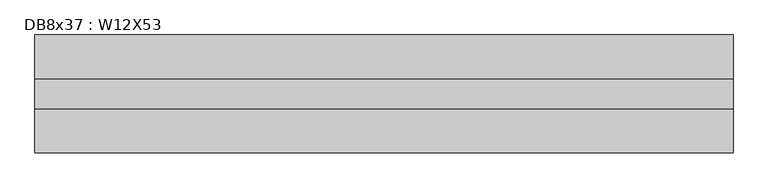
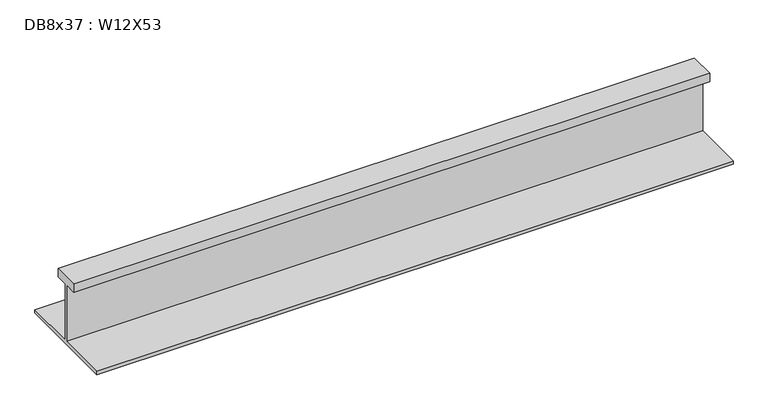
"""IFC4 building model written with IfcOpenShell, lengths in millimetres: beam geometry, DB8x37 : W12X53."""

import ifcopenshell
import ifcopenshell.guid

model = None  # the IFC model being written
_history = None  # IfcOwnerHistory: only IFC2X3 demands one
_inside = {}  # id of a spatial element -> (the spatial element, [elements in it])
_under = {}  # id of a project, library or spatial element -> (it, [spatial elements below it])
_declared = {}  # id of a project -> (the project, [libraries it declares])
_typed = {}  # id of a type object -> (the type object, [elements of that type])
_made_of = {}  # id of a material, layer set ... -> (it, [elements and type objects made of it])


def new_model(schema):
    """Start an empty IFC model of exactly this schema.

    Asked for "IFC4X3", IfcOpenShell would pick the latest addendum, in which some entities
    have other attributes; the version numbers below select the first issue.
    IFC2X3 requires an IfcOwnerHistory on every rooted entity: one is made here for all.
    """
    global model, _history
    if schema == "IFC4X3":
        model = ifcopenshell.file(schema_version=(4, 3, 0, 0))
    else:
        model = ifcopenshell.file(schema=schema)
    _inside.clear()
    _under.clear()
    _declared.clear()
    _typed.clear()
    _made_of.clear()
    _history = None
    if model.schema == "IFC2X3":
        org = make("IfcOrganization", Name="unknown")
        user = make(
            "IfcPersonAndOrganization",
            ThePerson=make("IfcPerson", FamilyName="unknown"),
            TheOrganization=org,
        )
        app = make(
            "IfcApplication",
            ApplicationDeveloper=org,
            Version="unknown",
            ApplicationFullName="unknown",
            ApplicationIdentifier="unknown",
        )
        _history = make(
            "IfcOwnerHistory",
            OwningUser=user,
            OwningApplication=app,
            ChangeAction="ADDED",
            CreationDate=0,
        )
    return model


def make(cls, **values):
    """One entity of the class cls with the attributes given. An attribute that is None is left unset."""
    return model.create_entity(
        cls, **{name: value for name, value in values.items() if value is not None}
    )


def rooted(cls, **values):
    """An entity with a GlobalId (a new one), such as an element, a storey or a relation."""
    return make(cls, GlobalId=ifcopenshell.guid.new(), OwnerHistory=_history, **values)


def si_unit(unit_type, name, prefix=None):
    """IfcSIUnit, for example si_unit("LENGTHUNIT", "METRE", prefix="MILLI")."""
    return make("IfcSIUnit", UnitType=unit_type, Prefix=prefix, Name=name)


def assignment(units):
    """IfcUnitAssignment: the units of a project."""
    return None if units is None else make("IfcUnitAssignment", Units=units)


def point(xyz):
    """IfcCartesianPoint."""
    return None if xyz is None else make("IfcCartesianPoint", Coordinates=xyz)


def direction(xyz):
    """IfcDirection."""
    return None if xyz is None else make("IfcDirection", DirectionRatios=xyz)


def frame(location, z_axis=None, x_axis=None):
    """IfcAxis2Placement3D, a coordinate frame: its origin and axes. An axis left out is left unset."""
    return make(
        "IfcAxis2Placement3D",
        Location=point(location),
        Axis=direction(z_axis),
        RefDirection=direction(x_axis),
    )


def origin():
    """The frame at (0, 0, 0) with its axes left unset."""
    return frame((0.0, 0.0, 0.0))


def place(relative_to, where):
    """IfcLocalPlacement: puts the frame where relative to a parent placement (None: the world)."""
    return make(
        "IfcLocalPlacement", PlacementRelTo=relative_to, RelativePlacement=where
    )


def context(
    kind, dimensions, precision=None, world=None, true_north=None, identifier=None
):
    """IfcGeometricRepresentationContext, for example the 3D "Model" context."""
    return make(
        "IfcGeometricRepresentationContext",
        ContextIdentifier=identifier,
        ContextType=kind,
        CoordinateSpaceDimension=dimensions,
        Precision=precision,
        WorldCoordinateSystem=world,
        TrueNorth=true_north,
    )


def project(units=None, contexts=None):
    """IfcProject with its units and contexts."""
    return rooted(
        "IfcProject",
        Name="project",
        RepresentationContexts=contexts,
        UnitsInContext=assignment(units),
    )


def spatial(cls, under=None, at=None, **own):
    """A site, building, storey or space (cls), placed at a placement, below another one or the project."""
    s = rooted(cls, ObjectPlacement=at, **own)
    if under is not None:
        _under.setdefault(under.id(), (under, []))[1].append(s)
    return s


def polyline(points):
    """IfcPolyline through the points."""
    return make("IfcPolyline", Points=[point(p) for p in points])


def outline(outer, holes=None, kind="AREA"):
    """IfcArbitraryClosedProfileDef: a profile drawn as a closed curve; with holes, ...WithVoids."""
    if holes is None:
        return make("IfcArbitraryClosedProfileDef", ProfileType=kind, OuterCurve=outer)
    return make(
        "IfcArbitraryProfileDefWithVoids",
        ProfileType=kind,
        OuterCurve=outer,
        InnerCurves=holes,
    )


def extrude(swept, where, along, depth):
    """IfcExtrudedAreaSolid: the profile swept, set in the frame where, extruded along a direction by depth."""
    return make(
        "IfcExtrudedAreaSolid",
        SweptArea=swept,
        Position=where,
        ExtrudedDirection=direction(along),
        Depth=depth,
    )


def shape(context_of_items, identifier, shape_type, items):
    """IfcShapeRepresentation: the items that make up one representation, for example the "Body"."""
    return make(
        "IfcShapeRepresentation",
        ContextOfItems=context_of_items,
        RepresentationIdentifier=identifier,
        RepresentationType=shape_type,
        Items=items,
    )


def source(mapping_origin, context_of_items, identifier, shape_type, items):
    """IfcRepresentationMap: a shape defined once, which mapped items show again and again."""
    return make(
        "IfcRepresentationMap",
        MappingOrigin=mapping_origin,
        MappedRepresentation=shape(context_of_items, identifier, shape_type, items),
    )


def transform(
    local_origin,
    x_axis=None,
    y_axis=None,
    z_axis=None,
    scale=None,
    scale2=None,
    scale3=None,
    uniform=True,
):
    """IfcCartesianTransformationOperator3D, or its non-uniform kind. x_axis, y_axis, z_axis: its Axis1, 2, 3."""
    if uniform:
        return make(
            "IfcCartesianTransformationOperator3D",
            Axis1=direction(x_axis),
            Axis2=direction(y_axis),
            LocalOrigin=point(local_origin),
            Scale=scale,
            Axis3=direction(z_axis),
        )
    return make(
        "IfcCartesianTransformationOperator3DnonUniform",
        Axis1=direction(x_axis),
        Axis2=direction(y_axis),
        LocalOrigin=point(local_origin),
        Scale=scale,
        Axis3=direction(z_axis),
        Scale2=scale2,
        Scale3=scale3,
    )


def mapped(mapping_source, mapping_target):
    """IfcMappedItem: shows the shape of a source again, moved by a transform."""
    return make(
        "IfcMappedItem", MappingSource=mapping_source, MappingTarget=mapping_target
    )


def made_of(thing, what):
    """Note that an element or type object is made of a material, layer set ...; save() writes the relation."""
    if what is not None:
        _made_of.setdefault(what.id(), (what, []))[1].append(thing)
    return thing


def element(
    cls,
    number,
    at=None,
    inside=None,
    cuts=None,
    type_object=None,
    material=None,
    context=None,
    identifier="Body",
    shape_type=None,
    held_by="IfcProductDefinitionShape",
    body=None,
    shapes=None,
    **own,
):
    """One element of the class cls, such as IfcWall. Its Tag is "e" and its number.

    at: its placement. inside: the storey or other place that contains it. cuts: it is an
    opening in that element (IfcRelVoidsElement). A single representation is given by context,
    identifier, shape_type and body (its items); several are given by shapes. held_by: the class
    of the entity that holds the representations. save() writes the other relations.
    """
    e = rooted(cls, Tag="e%d" % number, ObjectPlacement=at, **own)
    if body is not None:
        shapes = [shape(context, identifier, shape_type, body)]
    if shapes is not None:
        e.Representation = make(held_by, Representations=shapes)
    if inside is not None:
        _inside.setdefault(inside.id(), (inside, []))[1].append(e)
    if cuts is not None:
        rooted(
            "IfcRelVoidsElement", RelatingBuildingElement=cuts, RelatedOpeningElement=e
        )
    if type_object is not None:
        _typed.setdefault(type_object.id(), (type_object, []))[1].append(e)
    return made_of(e, material)


def aggregate(whole, parts):
    """IfcRelAggregates: a whole, such as a stair, and the parts it consists of."""
    return rooted("IfcRelAggregates", RelatingObject=whole, RelatedObjects=parts)


def save(model, path):
    """Write the relations noted so far, then the file.

    IfcRelAggregates (storeys below a building ...), IfcRelContainedInSpatialStructure (elements
    in a storey), IfcRelDefinesByType, IfcRelAssociatesMaterial and IfcRelDeclares: one each for
    every whole, place, type object, material and project.
    """
    for whole, parts in _under.values():
        aggregate(whole, parts)
    for where, things in _inside.values():
        rooted(
            "IfcRelContainedInSpatialStructure",
            RelatedElements=things,
            RelatingStructure=where,
        )
    for kind, things in _typed.values():
        rooted("IfcRelDefinesByType", RelatedObjects=things, RelatingType=kind)
    for what, things in _made_of.values():
        rooted("IfcRelAssociatesMaterial", RelatedObjects=things, RelatingMaterial=what)
    for by, libraries in _declared.values():
        rooted("IfcRelDeclares", RelatingContext=by, RelatedDefinitions=libraries)
    model.write(path)


def db8x37_w12x53_300c3b95(model_context):
    return source(origin(), model_context, "Body", "SweptSolid", [
        extrude(outline(polyline([(38.1, 145.415), (38.1, 120.015), (2.921, 120.015), (2.921, -48.4505), (152.4, -48.4505), (152.4, -58.1025), (-152.4, -58.1025), (-152.4, -48.4505), (-2.921, -48.4505), (-2.921, 120.015), (-38.1, 120.015), (-38.1, 145.415), (38.1, 145.415)])), frame((-851.408, 0.0, 0.0), z_axis=(1.0, 0.0, 0.0), x_axis=(0.0, 1.0, 0.0)), (0.0, 0.0, 1.0), 1803.9079994),
    ])


if __name__ == "__main__":
    model = new_model("IFC4")
    model_context = context("Model", 3, world=origin())
    ifc_project = project(units=[si_unit("LENGTHUNIT", "METRE", prefix="MILLI")], contexts=[model_context])
    site = spatial("IfcSite", under=ifc_project)
    building = spatial("IfcBuilding", under=site)
    placement = place(None, origin())
    db8x37_w12x53_shape = db8x37_w12x53_300c3b95(model_context)
    element("IfcBeam", 1, ObjectType="DB8x37 : W12X53", at=placement, inside=building, context=model_context, shape_type="MappedRepresentation", body=[
        mapped(db8x37_w12x53_shape, transform((0.0, 0.0, 0.0), x_axis=(1.0, 0.0, 0.0), y_axis=(0.0, 1.0, 0.0), z_axis=(0.0, 0.0, 1.0))),
    ])
    save(model, "model.ifc")

# Revit data of these elements
# Type "DB8x37 : W12X53"
#   Assembly Code = "B10"
#   W = 53
#   Length [instance default] = 5' - 0"
#   bf = 0' - 10"
#   d = 1' - 0.1"
#   k = 0' - 1 3/8"
#   k2 = 0' - 0.8"
#   tf = 0' - 0.575"
#   tw = 0' - 0.345"
#   A = 0.108333 SF
#   Structural Material [instance default] = Steel ASTM A992
# Element 1 (IfcBeam, "DB8x37 : W12X53")
#   Materials on its faces: "Steel ASTM A992"
# Materials
#   "Steel ASTM A992": class "Metal", colour RGB 199 199 199, transparency 0, Description = "Structural steel 50ksi", Cost = 0
